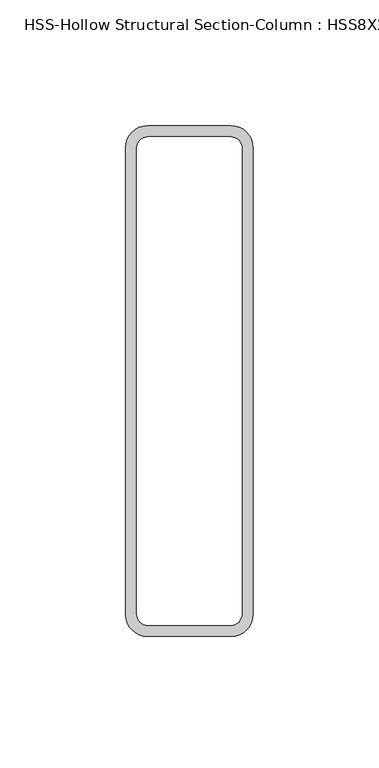
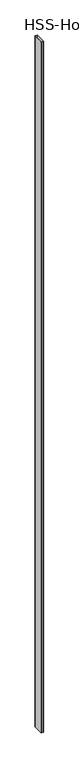
"""IFC4 building model written with IfcOpenShell, lengths in millimetres: column geometry, HSS-Hollow Structural Section-Column : HSS8X2X3/16."""

from ifc_helpers import new_model, si_unit, point, frame, frame_2d, origin, place, context, project, spatial, polyline, circle_curve, trimmed, segment, composite_curve, outline, extrude, source, transform, mapped, element, save


def hss_hollow_structural_section_column_hss8x2x3_16_deeb36db(model_context):
    return source(origin(), model_context, "Body", "SweptSolid", [
        extrude(outline(composite_curve([segment(trimmed(circle_curve(frame_2d((16.5608, 92.7608)), 8.8392), [point((16.5608, 101.6))], [point((25.4, 92.7608))], False, "CARTESIAN"), True, "CONTINUOUS"), segment(polyline([(25.4, 92.7608), (25.4, -92.7608)]), True, "CONTINUOUS"), segment(trimmed(circle_curve(frame_2d((16.5608, -92.7608)), 8.8392), [point((25.4, -92.7608))], [point((16.5608, -101.6))], False, "CARTESIAN"), True, "CONTINUOUS"), segment(polyline([(16.5608, -101.6), (-16.5608, -101.6)]), True, "CONTINUOUS"), segment(trimmed(circle_curve(frame_2d((-16.5608, -92.7608)), 8.8392), [point((-16.5608, -101.6))], [point((-25.4, -92.7608))], False, "CARTESIAN"), True, "CONTINUOUS"), segment(polyline([(-25.4, -92.7608), (-25.4, 92.7608)]), True, "CONTINUOUS"), segment(trimmed(circle_curve(frame_2d((-16.5608, 92.7608)), 8.8392), [point((-25.4, 92.7608))], [point((-16.5608, 101.6))], False, "CARTESIAN"), True, "CONTINUOUS"), segment(polyline([(-16.5608, 101.6), (16.5608, 101.6)]), True, "CONTINUOUS")], self_intersect=False), holes=[composite_curve([segment(polyline([(16.5608, 97.1804), (-16.5608, 97.1804)]), True, "CONTINUOUS"), segment(trimmed(circle_curve(frame_2d((-16.5608, 92.7608)), 4.4196), [point((-16.5608, 97.1804))], [point((-20.9804, 92.7608))], True, "CARTESIAN"), True, "CONTINUOUS"), segment(polyline([(-20.9804, 92.7608), (-20.9804, -92.7608)]), True, "CONTINUOUS"), segment(trimmed(circle_curve(frame_2d((-16.5608, -92.7608)), 4.4196), [point((-20.9804, -92.7608))], [point((-16.5608, -97.1804))], True, "CARTESIAN"), True, "CONTINUOUS"), segment(polyline([(-16.5608, -97.1804), (16.5608, -97.1804)]), True, "CONTINUOUS"), segment(trimmed(circle_curve(frame_2d((16.5608, -92.7608)), 4.4196), [point((16.5608, -97.1804))], [point((20.9804, -92.7608))], True, "CARTESIAN"), True, "CONTINUOUS"), segment(polyline([(20.9804, -92.7608), (20.9804, 92.7608)]), True, "CONTINUOUS"), segment(trimmed(circle_curve(frame_2d((16.5608, 92.7608)), 4.4196), [point((20.9804, 92.7608))], [point((16.5608, 97.1804))], True, "CARTESIAN"), True, "CONTINUOUS")], self_intersect=False)]), frame((0.0, 0.0, -350.0), z_axis=(0.0, 0.0, 1.0), x_axis=(1.0, 0.0, 0.0)), (0.0, 0.0, 1.0), 13350.0),
    ])


if __name__ == "__main__":
    model = new_model("IFC4")
    model_context = context("Model", 3, world=origin())
    ifc_project = project(units=[si_unit("LENGTHUNIT", "METRE", prefix="MILLI")], contexts=[model_context])
    site = spatial("IfcSite", under=ifc_project)
    building = spatial("IfcBuilding", under=site)
    placement = place(None, origin())
    hss_hollow_structural_section_column_hss8x2x3_16_shape = hss_hollow_structural_section_column_hss8x2x3_16_deeb36db(model_context)
    element("IfcColumn", 1, ObjectType="HSS-Hollow Structural Section-Column : HSS8X2X3/16", at=placement, inside=building, context=model_context, shape_type="MappedRepresentation", body=[
        mapped(hss_hollow_structural_section_column_hss8x2x3_16_shape, transform((0.0, 0.0, 0.0), x_axis=(1.0, 0.0, 0.0), y_axis=(0.0, 1.0, 0.0), z_axis=(0.0, 0.0, 1.0))),
    ])
    save(model, "model.ifc")

# Revit data of these elements
# Type "HSS-Hollow Structural Section-Column : HSS8X2X3/16"
#   Assembly Code = "B10"
#   Shape = "Rect."
#   Cost = 1
#   W = 12
#   Ht = 203.2 mm
#   b = 50.8 mm
#   kr = 8.839 mm
#   t = 4.42 mm
#   A = 0.00211612 m²
#   Structural Material [instance default] = Steel ASTM A500, Grade B, Rectangular and Square
# Element 1 (IfcColumn, "HSS-Hollow Structural Section-Column : HSS8X2X3/16")
#   Structural Material = Metal - Steel 43-275
#   Materials on its faces: "Metal - Steel 43-275"
# Materials
#   "Steel ASTM A500, Grade B, Rectangular and Square": class "Metal", colour RGB 199 199 199, transparency 0, Description = "Carbon steel", Cost = 0
#   "Metal - Steel 43-275": class "Metal", colour RGB 247 247 247, transparency 0, Cost = 0
